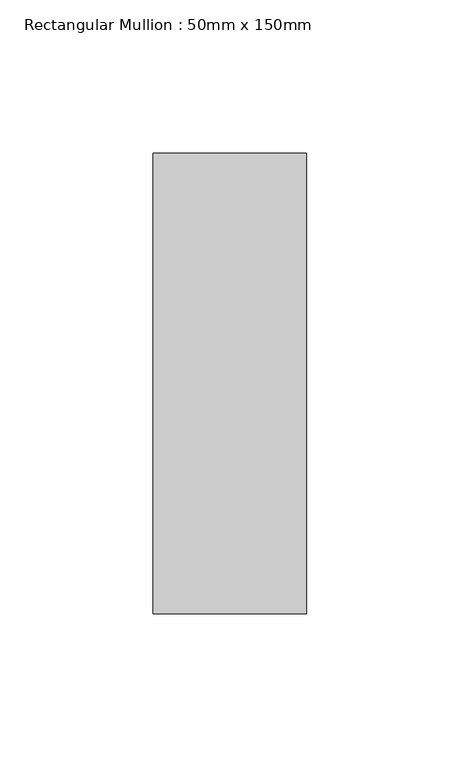
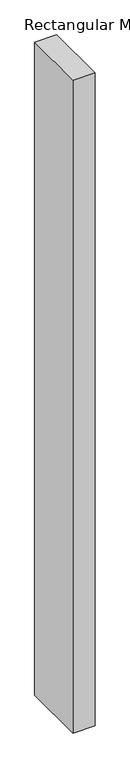
"""IFC4 building model written with IfcOpenShell, lengths in millimetres: member geometry, Rectangular Mullion : 50mm x 150mm."""

from ifc_helpers import new_model, si_unit, frame, origin, place, context, project, spatial, polyline, outline, extrude, source, transform, mapped, element, save


def rectangular_mullion_50mm_x_150mm_6a25db57(model_context):
    return source(origin(), model_context, "Body", "SweptSolid", [
        extrude(outline(polyline([(0.0, 75.0), (0.0, -75.0), (-50.0, -75.0), (-50.0, 75.0), (0.0, 75.0)])), frame((0.0, 0.0, -1565.6357052), z_axis=(0.0, 0.0, 1.0), x_axis=(1.0, 0.0, 0.0)), (0.0, 0.0, 1.0), 1565.6357052),
    ])


if __name__ == "__main__":
    model = new_model("IFC4")
    model_context = context("Model", 3, world=origin())
    ifc_project = project(units=[si_unit("LENGTHUNIT", "METRE", prefix="MILLI")], contexts=[model_context])
    site = spatial("IfcSite", under=ifc_project)
    building = spatial("IfcBuilding", under=site)
    placement = place(None, origin())
    rectangular_mullion_50mm_x_150mm_shape = rectangular_mullion_50mm_x_150mm_6a25db57(model_context)
    element("IfcMember", 1, ObjectType="Rectangular Mullion : 50mm x 150mm", at=placement, inside=building, context=model_context, shape_type="MappedRepresentation", body=[
        mapped(rectangular_mullion_50mm_x_150mm_shape, transform((0.0, 0.0, 0.0), x_axis=(1.0, 0.0, 0.0), y_axis=(0.0, 1.0, 0.0), z_axis=(0.0, 0.0, 1.0))),
    ])
    save(model, "model.ifc")

# Revit data of these elements
# Type "Rectangular Mullion : 50mm x 150mm"
#   built-in parameter 1007304 = 0.492126 (stored number, unit not read)
#   built-in parameter 1007301 = 0.082021 (stored number, unit not read)
#   built-in parameter 1007300 = 0.082021 (stored number, unit not read)
# Element 1 (IfcMember, "Rectangular Mullion : 50mm x 150mm")
#   Materials on its faces: "Aluminum"
# Materials
#   "Aluminum": class "Metal", colour RGB 244 244 244, transparency 0, Description = "Aluminum 6061", Cost = 0
